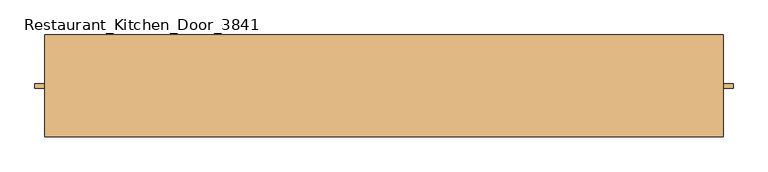
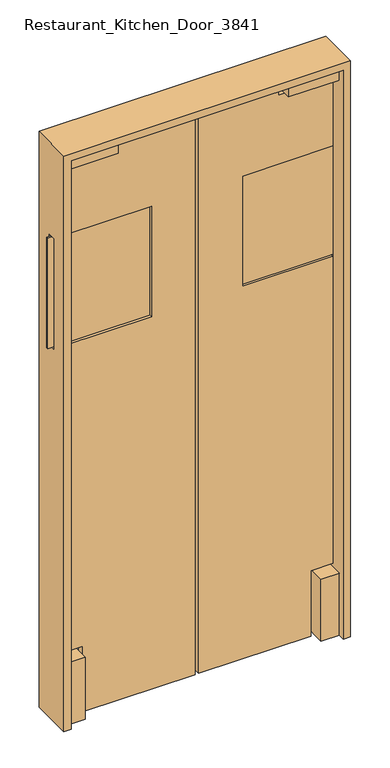
"""IFC4 building model written with IfcOpenShell, lengths in millimetres: door geometry, Restaurant_Kitchen_Door_3841."""

from ifc_helpers import new_model, si_unit, frame, origin, origin_with_axes, place, context, project, spatial, polyline, outline, extrude, faceted_brep, source, transform, mapped, element, save


def restaurant_kitchen_door_3841_1d1f979e(model_context):
    return source(origin(), model_context, "Body", "SolidModel", [
        faceted_brep([(-500.0, -75.0, 0.0), (-500.0, 75.0, 0.0), (-474.6, 75.0, 0.0), (-474.6, -75.0, 0.0), (-500.0, -75.0, 2120.0), (-500.0, 75.0, 2120.0), (-500.0, -12.7, 1778.0), (-500.0, -12.7, 1371.6), (-500.0, 12.7, 1371.6), (-500.0, 12.7, 1778.0), (500.0, 75.0, 2120.0), (500.0, 75.0, 0.0), (474.6, 75.0, 0.0), (474.6, 75.0, 2094.6), (-474.6, 75.0, 2094.6), (-474.6, -75.0, 2094.6), (-474.6, -12.7, 1371.6), (-474.6, -12.7, 1778.0), (-474.6, 12.7, 1778.0), (-474.6, 12.7, 1371.6), (474.6, -75.0, 2094.6), (474.6, -75.0, 0.0), (500.0, -75.0, 0.0), (500.0, -75.0, 2120.0), (500.0, 12.7, 1778.0), (500.0, 12.7, 1371.6), (500.0, -12.7, 1371.6), (500.0, -12.7, 1778.0), (474.6, 12.7, 1371.6), (474.6, 12.7, 1778.0), (474.6, -12.7, 1778.0), (474.6, -12.7, 1371.6)], [[[0, 1, 2, 3]], [[1, 0, 4, 5], [6, 7, 8, 9]], [[2, 1, 5, 10, 11, 12, 13, 14]], [[3, 2, 14, 15], [16, 17, 18, 19]], [[0, 3, 15, 20, 21, 22, 23, 4]], [[11, 10, 23, 22], [24, 25, 26, 27]], [[12, 11, 22, 21]], [[13, 12, 21, 20], [28, 29, 30, 31]], [[5, 4, 23, 10]], [[14, 13, 20, 15]], [[30, 27, 26, 31]], [[28, 25, 24, 29]], [[25, 28, 31, 26]], [[29, 24, 27, 30]], [[16, 7, 6, 17]], [[18, 9, 8, 19]], [[17, 6, 9, 18]], [[7, 16, 19, 8]]]),
        extrude(outline(polyline([(-296.8, -50.8), (-474.6, -50.8), (-474.6, 50.8), (-296.8, 50.8), (-296.8, -50.8)])), frame((0.0, 0.0, 2043.8), z_axis=(0.0, 0.0, 1.0), x_axis=(1.0, 0.0, 0.0)), (0.0, 0.0, 1.0), 50.8),
        extrude(outline(polyline([(474.6, -50.8), (296.8, -50.8), (296.8, 50.8), (474.6, 50.8), (474.6, -50.8)])), frame((0.0, 0.0, 2043.8), z_axis=(0.0, 0.0, 1.0), x_axis=(1.0, 0.0, 0.0)), (0.0, 0.0, 1.0), 50.8),
        extrude(outline(polyline([(474.6, -50.8), (411.1, -50.8), (411.1, 50.8), (474.6, 50.8), (474.6, -50.8)])), origin_with_axes(), (0.0, 0.0, 1.0), 228.6),
        extrude(outline(polyline([(-411.1, -50.8), (-474.6, -50.8), (-474.6, 50.8), (-411.1, 50.8), (-411.1, -50.8)])), origin_with_axes(), (0.0, 0.0, 1.0), 228.6),
        extrude(outline(polyline([(-158.75, -3.175), (-514.35, -3.175), (-514.35, 3.175), (-158.75, 3.175), (-158.75, -3.175)])), frame((0.0, 0.0, 1371.6), z_axis=(0.0, 0.0, 1.0), x_axis=(1.0, 0.0, 0.0)), (0.0, 0.0, 1.0), 406.4),
        extrude(outline(polyline([(241.3, -474.6), (241.3, -398.4), (0.0, -398.4), (0.0, -6.35), (2094.6, -6.35), (2094.6, -284.1), (2031.1, -284.1), (2031.1, -474.6), (1778.0, -474.6), (1778.0, -158.75), (1371.6, -158.75), (1371.6, -474.6), (241.3, -474.6)])), frame((0.0, -12.7, 0.0), z_axis=(0.0, 1.0, 0.0), x_axis=(0.0, 0.0, 1.0)), (0.0, 0.0, 1.0), 25.4),
        extrude(outline(polyline([(514.35, -3.175), (158.75, -3.175), (158.75, 3.175), (514.35, 3.175), (514.35, -3.175)])), frame((0.0, 0.0, 1371.6), z_axis=(0.0, 0.0, 1.0), x_axis=(1.0, 0.0, 0.0)), (0.0, 0.0, 1.0), 406.4),
        extrude(outline(polyline([(2031.1, 474.6), (2031.1, 284.1), (2094.6, 284.1), (2094.6, 6.35), (0.0, 6.35), (0.0, 398.4), (241.3, 398.4), (241.3, 474.6), (1371.6, 474.6), (1371.6, 158.75), (1778.0, 158.75), (1778.0, 474.6), (2031.1, 474.6)])), frame((0.0, -12.7, 0.0), z_axis=(0.0, 1.0, 0.0), x_axis=(0.0, 0.0, 1.0)), (0.0, 0.0, 1.0), 25.4),
    ])


if __name__ == "__main__":
    model = new_model("IFC4")
    model_context = context("Model", 3, world=origin())
    ifc_project = project(units=[si_unit("LENGTHUNIT", "METRE", prefix="MILLI")], contexts=[model_context])
    site = spatial("IfcSite", under=ifc_project)
    building = spatial("IfcBuilding", under=site)
    placement = place(None, origin())
    restaurant_kitchen_door_3841_shape = restaurant_kitchen_door_3841_1d1f979e(model_context)
    element("IfcDoor", 1, ObjectType="Restaurant_Kitchen_Door_3841 : 5'-4\"W. x 7'-2\"H. 22", at=placement, inside=building, context=model_context, shape_type="MappedRepresentation", body=[
        mapped(restaurant_kitchen_door_3841_shape, transform((0.0, 0.0, 0.0), x_axis=(1.0, 0.0, 0.0), y_axis=(0.0, 1.0, 0.0), z_axis=(0.0, 0.0, 1.0))),
    ])
    save(model, "model.ifc")

# Revit data of these elements
# Project information
#   Project Issue Date = "Issue Date"
#   Project Status = "Project Status"
#   Client Name = "Owner"
#   Project Address = "Enter address here"
#   Project Name = "Project Name"
#   Project Number = "Project Number"
# Type "Restaurant_Kitchen_Door_3841 : 5'-4\"W. x 7'-2\"H. 22"
#   Type Mark = "C27"
#   Analytic Construction = "<Nenhum>"
#   Rough Width = 1000 mm
#   Rough Height = 2120 mm
#   Height = 2094.6 mm
#   Width = 474.6 mm
#   Define Thermal Properties by = 1
#   Glass = Glazing - Interior
#   Frame = Door - Kitchen - Frame
#   Door Panel = Door - Kitchen - Panel
#   Function = (empty or 0)
#   Wall Closure = (empty or 0)
# Element 1 (IfcDoor, "Restaurant_Kitchen_Door_3841 : 5'-4\"W. x 7'-2\"H. 22")
#   Materials on its faces: "Door - Kitchen - Frame", "Door - Kitchen - Panel", "Glazing - Interior"
# Materials
#   "Glazing - Interior": class "Não atribuído", colour RGB 0 0 255, transparency 0.75
#   "Door - Kitchen - Frame": class "Não atribuído", colour RGB 247 247 247, transparency 0
#   "Door - Kitchen - Panel": class "Não atribuído", colour RGB 50 50 50, transparency 0, Comments = "A aparência de renderização não foi atualizada "
